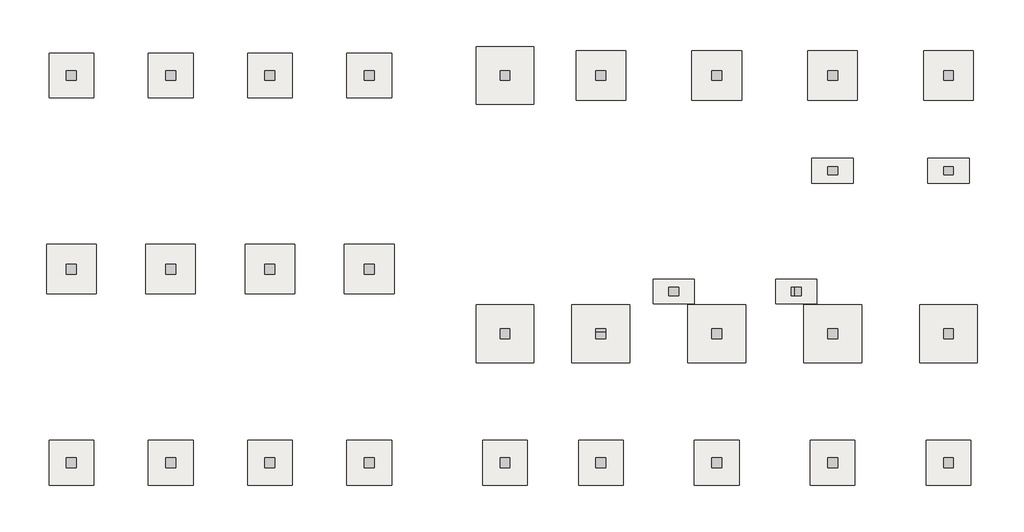
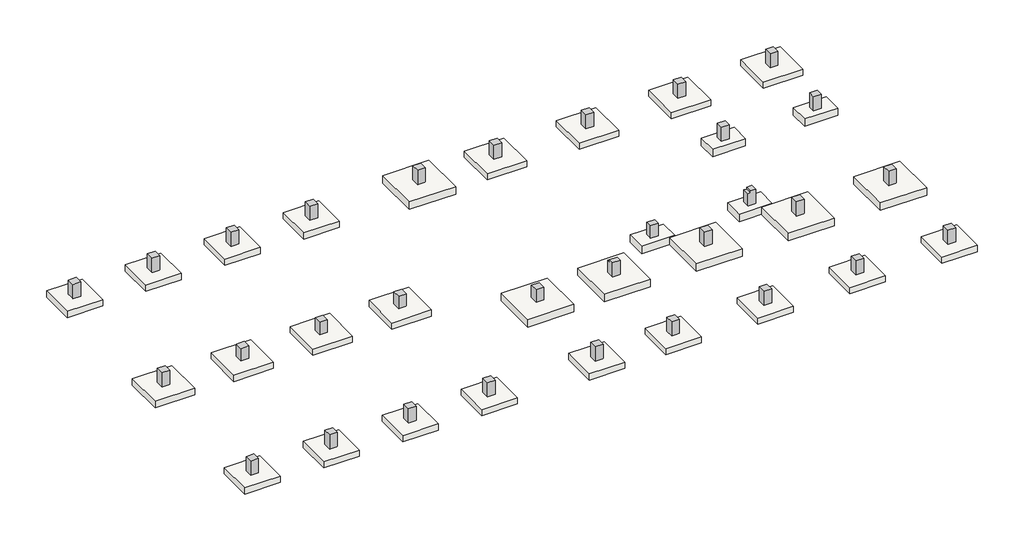
# Not in any storey: 31 columns, 31 slabs.
# Revit data of these elements (continued)
# Type "Foundation Rectangular (Non-Pile) : H_SF_AR_S18_W2700xL2700xT500_Bitumen_F1" (continued)
#   H_WM Code_1 = "A03AD032-00010 |  | M3 | Concrete Work | Substructure Work | Structural Concrete | Cement Type-1 | 20MPa < F'c (Cylinder Strength) ≤ 25MPa |  |  |  | A03AD032-00010 Concrete Work Substructure Work Structural Concrete  Cement Type-1 20MPa < F'c (Cylinder Strength) ≤ 25MPa      |  F'c (Cylinder Strength) = 24MPa"
#   H_WM Code_2 = "A03AD037-00002 |  | TON | Concrete Work | Substructure Work | Rebar Work | Deformed Bar (Non-Coat.) | 400MPa<Fy≤470MPa |  |  |  | A03AD037-00002 Concrete Work Substructure Work Rebar Work Deformed Bar (Non-Coat.)  400MPa<Fy≤470MPa      | ASTM A615 GRADE 60 (Fy=420MPa)"
#   H_WM Code_3 = "A03AD035-00001 |  | M2 | Concrete Work | Substructure Work | Form Work (3 times in use) | Flat Form | Dressed Lumber, Plywood or Steel Form(Wood Planks are not Allowed) incl. Chamfer |  |  | A03AD035-00001 Concrete Work Substructure Work Form Work (3 times in use) Flat Form     Dressed Lumber, Plywood or Steel Form(Wood Planks are not Allowed) incl. Chamfer   |"
#   H_WM Code_4 = "A03AH056-00001 |  | M2 | Concrete Work | Concrete Protective Coating (U/G) | Bitumen/Bituminous/Asphalt Coating |  | A03AH056-00001 Concrete Work Concrete Protective Coating (U/G) Bitumen/Bituminous/Asphalt Coating         |"
#   H_WM Code_5 = "A01ZZ001-00004 |  | M3 | Earth Work | - | Excavation | Soil, Mech. |  | D ≤ 2.0M |  |  | A01ZZ001-00004 Earth Work - Excavation Soil, Mech.      D ≤ 2.0M  | D=2.0m"
#   H_WM Code_6 = "A01ZZ003-00001 |  | M3 | Earth Work | - | Backfill | Re-use, Soil |  |  |  | Compaction=(  )% | A01ZZ003-00001 Earth Work - Backfill Re-use, Soil        | Compaction=( 95 )%"
#   H_WM Code_7 = "A01ZZ004-00001 |  | M3 | Earth Work | - | Disposal | Soil |  |  |  | Disposal Distance=Appx. (  )km from Site | A01ZZ004-00001 Earth Work - Disposal Soil        | Disposal Distance=Appx. (20 )km from Site"
#   Top bar = "D25@300"
#   Description = "UG Shallow Foundation"
#   Bottom bar = "D20@300"
#   Width = 2700 mm
#   Length = 2700 mm
#   Foundation Thickness = 500 mm
#   Structural Material [instance default] = none
#   Assembly Code = ""
# Type "Foundation Rectangular (Non-Pile) : H_SF_AR_S18_W3500xL3500xT600_Bitumen_F3"
#   H_Q'ty Cal Type Tag = "SF-Q4"
#   H_WM Code_1 = "A03AD032-00010 |  | M3 | Concrete Work | Substructure Work | Structural Concrete | Cement Type-1 | 20MPa < F'c (Cylinder Strength) ≤ 25MPa |  |  |  | A03AD032-00010 Concrete Work Substructure Work Structural Concrete  Cement Type-1 20MPa < F'c (Cylinder Strength) ≤ 25MPa      |  F'c (Cylinder Strength) = 24MPa"
#   H_WM Code_2 = "A03AD037-00002 |  | TON | Concrete Work | Substructure Work | Rebar Work | Deformed Bar (Non-Coat.) | 400MPa<Fy≤470MPa |  |  |  | A03AD037-00002 Concrete Work Substructure Work Rebar Work Deformed Bar (Non-Coat.)  400MPa<Fy≤470MPa      | ASTM A615 GRADE 60 (Fy=420MPa)"
#   H_WM Code_3 = "A03AD035-00001 |  | M2 | Concrete Work | Substructure Work | Form Work (3 times in use) | Flat Form | Dressed Lumber, Plywood or Steel Form(Wood Planks are not Allowed) incl. Chamfer |  |  | A03AD035-00001 Concrete Work Substructure Work Form Work (3 times in use) Flat Form     Dressed Lumber, Plywood or Steel Form(Wood Planks are not Allowed) incl. Chamfer   |"
#   H_WM Code_4 = "A03AH056-00001 |  | M2 | Concrete Work | Concrete Protective Coating (U/G) | Bitumen/Bituminous/Asphalt Coating |  | A03AH056-00001 Concrete Work Concrete Protective Coating (U/G) Bitumen/Bituminous/Asphalt Coating         |"
#   H_WM Code_5 = "A01ZZ001-00004 |  | M3 | Earth Work | - | Excavation | Soil, Mech. |  | D ≤ 2.0M |  |  | A01ZZ001-00004 Earth Work - Excavation Soil, Mech.      D ≤ 2.0M  | D=2.0m"
#   H_WM Code_6 = "A01ZZ003-00001 |  | M3 | Earth Work | - | Backfill | Re-use, Soil |  |  |  | Compaction=(  )% | A01ZZ003-00001 Earth Work - Backfill Re-use, Soil        | Compaction=( 95 )%"
#   H_WM Code_7 = "A01ZZ004-00001 |  | M3 | Earth Work | - | Disposal | Soil |  |  |  | Disposal Distance=Appx. (  )km from Site | A01ZZ004-00001 Earth Work - Disposal Soil        | Disposal Distance=Appx. (20 )km from Site"
#   Top bar = "D25@300"
#   Description = "UG Shallow Foundation"
#   Bottom bar = "D20@300"
#   Width = 3500 mm
#   Length = 3500 mm
#   Foundation Thickness = 600 mm
#   Structural Material [instance default] = none
#   Assembly Code = ""
# Type "Foundation Rectangular (Non-Pile) : H_SF_AR_S18_W3000xL3000xT500_Bitumen_F2A"
#   H_Q'ty Cal Type Tag = "SF-Q4"
#   H_WM Code_1 = "A03AD032-00010 |  | M3 | Concrete Work | Substructure Work | Structural Concrete | Cement Type-1 | 20MPa < F'c (Cylinder Strength) ≤ 25MPa |  |  |  | A03AD032-00010 Concrete Work Substructure Work Structural Concrete  Cement Type-1 20MPa < F'c (Cylinder Strength) ≤ 25MPa      |  F'c (Cylinder Strength) = 24MPa"
#   H_WM Code_2 = "A03AD037-00002 |  | TON | Concrete Work | Substructure Work | Rebar Work | Deformed Bar (Non-Coat.) | 400MPa<Fy≤470MPa |  |  |  | A03AD037-00002 Concrete Work Substructure Work Rebar Work Deformed Bar (Non-Coat.)  400MPa<Fy≤470MPa      | ASTM A615 GRADE 60 (Fy=420MPa)"
#   H_WM Code_3 = "A03AD035-00001 |  | M2 | Concrete Work | Substructure Work | Form Work (3 times in use) | Flat Form | Dressed Lumber, Plywood or Steel Form(Wood Planks are not Allowed) incl. Chamfer |  |  | A03AD035-00001 Concrete Work Substructure Work Form Work (3 times in use) Flat Form     Dressed Lumber, Plywood or Steel Form(Wood Planks are not Allowed) incl. Chamfer   |"
#   H_WM Code_4 = "A03AH056-00001 |  | M2 | Concrete Work | Concrete Protective Coating (U/G) | Bitumen/Bituminous/Asphalt Coating |  | A03AH056-00001 Concrete Work Concrete Protective Coating (U/G) Bitumen/Bituminous/Asphalt Coating         |"
#   H_WM Code_5 = "A01ZZ001-00004 |  | M3 | Earth Work | - | Excavation | Soil, Mech. |  | D ≤ 2.0M |  |  | A01ZZ001-00004 Earth Work - Excavation Soil, Mech.      D ≤ 2.0M  | D=2.0m"
#   H_WM Code_6 = "A01ZZ003-00001 |  | M3 | Earth Work | - | Backfill | Re-use, Soil |  |  |  | Compaction=(  )% | A01ZZ003-00001 Earth Work - Backfill Re-use, Soil        | Compaction=( 95 )%"
#   H_WM Code_7 = "A01ZZ004-00001 |  | M3 | Earth Work | - | Disposal | Soil |  |  |  | Disposal Distance=Appx. (  )km from Site | A01ZZ004-00001 Earth Work - Disposal Soil        | Disposal Distance=Appx. (20 )km from Site"
#   Top bar = "D25@300"
#   Description = "UG Shallow Foundation"
#   Bottom bar = "D20@300"
#   Width = 3000 mm
#   Length = 3000 mm
#   Foundation Thickness = 500 mm
#   Structural Material [instance default] = none
#   Assembly Code = ""
# Type "Foundation Rectangular (Non-Pile) : H_SF_AR_S18_W2700xL2700xT500_Bitumen_F1A"
#   H_Q'ty Cal Type Tag = "SF-Q4"
#   H_WM Code_1 = "A03AD032-00010 |  | M3 | Concrete Work | Substructure Work | Structural Concrete | Cement Type-1 | 20MPa < F'c (Cylinder Strength) ≤ 25MPa |  |  |  | A03AD032-00010 Concrete Work Substructure Work Structural Concrete  Cement Type-1 20MPa < F'c (Cylinder Strength) ≤ 25MPa      |  F'c (Cylinder Strength) = 24MPa"
#   H_WM Code_2 = "A03AD037-00002 |  | TON | Concrete Work | Substructure Work | Rebar Work | Deformed Bar (Non-Coat.) | 400MPa<Fy≤470MPa |  |  |  | A03AD037-00002 Concrete Work Substructure Work Rebar Work Deformed Bar (Non-Coat.)  400MPa<Fy≤470MPa      | ASTM A615 GRADE 60 (Fy=420MPa)"
#   H_WM Code_3 = "A03AD035-00001 |  | M2 | Concrete Work | Substructure Work | Form Work (3 times in use) | Flat Form | Dressed Lumber, Plywood or Steel Form(Wood Planks are not Allowed) incl. Chamfer |  |  | A03AD035-00001 Concrete Work Substructure Work Form Work (3 times in use) Flat Form     Dressed Lumber, Plywood or Steel Form(Wood Planks are not Allowed) incl. Chamfer   |"
#   H_WM Code_4 = "A03AH056-00001 |  | M2 | Concrete Work | Concrete Protective Coating (U/G) | Bitumen/Bituminous/Asphalt Coating |  | A03AH056-00001 Concrete Work Concrete Protective Coating (U/G) Bitumen/Bituminous/Asphalt Coating         |"
#   H_WM Code_5 = "A01ZZ001-00004 |  | M3 | Earth Work | - | Excavation | Soil, Mech. |  | D ≤ 2.0M |  |  | A01ZZ001-00004 Earth Work - Excavation Soil, Mech.      D ≤ 2.0M  | D=2.0m"
#   H_WM Code_6 = "A01ZZ003-00001 |  | M3 | Earth Work | - | Backfill | Re-use, Soil |  |  |  | Compaction=(  )% | A01ZZ003-00001 Earth Work - Backfill Re-use, Soil        | Compaction=( 95 )%"
#   H_WM Code_7 = "A01ZZ004-00001 |  | M3 | Earth Work | - | Disposal | Soil |  |  |  | Disposal Distance=Appx. (  )km from Site | A01ZZ004-00001 Earth Work - Disposal Soil        | Disposal Distance=Appx. (20 )km from Site"
#   Top bar = "D25@300"
#   Description = "UG Shallow Foundation"
#   Bottom bar = "D20@300"
#   Width = 2700 mm
#   Length = 2700 mm
#   Foundation Thickness = 500 mm
#   Structural Material [instance default] = none
#   Assembly Code = ""
# Type "Foundation Rectangular (Non-Pile) : H_SF_AR_S18_W2500xL1500xT600_Bitumen_F4"
#   H_Q'ty Cal Type Tag = "SF-Q4"
#   H_WM Code_1 = "A03AD032-00010 |  | M3 | Concrete Work | Substructure Work | Structural Concrete | Cement Type-1 | 20MPa < F'c (Cylinder Strength) ≤ 25MPa |  |  |  | A03AD032-00010 Concrete Work Substructure Work Structural Concrete  Cement Type-1 20MPa < F'c (Cylinder Strength) ≤ 25MPa      |  F'c (Cylinder Strength) = 24MPa"
#   H_WM Code_2 = "A03AD037-00002 |  | TON | Concrete Work | Substructure Work | Rebar Work | Deformed Bar (Non-Coat.) | 400MPa<Fy≤470MPa |  |  |  | A03AD037-00002 Concrete Work Substructure Work Rebar Work Deformed Bar (Non-Coat.)  400MPa<Fy≤470MPa      | ASTM A615 GRADE 60 (Fy=420MPa)"
#   H_WM Code_3 = "A03AD035-00001 |  | M2 | Concrete Work | Substructure Work | Form Work (3 times in use) | Flat Form | Dressed Lumber, Plywood or Steel Form(Wood Planks are not Allowed) incl. Chamfer |  |  | A03AD035-00001 Concrete Work Substructure Work Form Work (3 times in use) Flat Form     Dressed Lumber, Plywood or Steel Form(Wood Planks are not Allowed) incl. Chamfer   |"
#   H_WM Code_4 = "A03AH056-00001 |  | M2 | Concrete Work | Concrete Protective Coating (U/G) | Bitumen/Bituminous/Asphalt Coating |  | A03AH056-00001 Concrete Work Concrete Protective Coating (U/G) Bitumen/Bituminous/Asphalt Coating         |"
#   H_WM Code_5 = "A01ZZ001-00004 |  | M3 | Earth Work | - | Excavation | Soil, Mech. |  | D ≤ 2.0M |  |  | A01ZZ001-00004 Earth Work - Excavation Soil, Mech.      D ≤ 2.0M  | D=2.0m"
#   H_WM Code_6 = "A01ZZ003-00001 |  | M3 | Earth Work | - | Backfill | Re-use, Soil |  |  |  | Compaction=(  )% | A01ZZ003-00001 Earth Work - Backfill Re-use, Soil        | Compaction=( 95 )%"
#   H_WM Code_7 = "A01ZZ004-00001 |  | M3 | Earth Work | - | Disposal | Soil |  |  |  | Disposal Distance=Appx. (  )km from Site | A01ZZ004-00001 Earth Work - Disposal Soil        | Disposal Distance=Appx. (20 )km from Site"
#   Top bar = "D25@300"
#   Description = "UG Shallow Foundation"
#   Bottom bar = "D20@300"
#   Width = 2500 mm
#   Length = 1500 mm
#   Foundation Thickness = 600 mm
#   Structural Material [instance default] = none
#   Assembly Code = ""
# Elements 1, 2, 3, 4, 5, 6, 7, 8, 9, 10, 11, 12, 13, 14, 15, 16, 17, 18, 19, 20, 21, 22, 23, 24, 25, 26, 27 (IfcColumn, "RC_Column_Rectangular : H_SC_AR_S15_UG PED_W600xL600_Bit")
#   Comments = ""
#   hec_material3 = none
#   hec_material2 = none
#   hec_material1 = none
#   Structural Material = Concrete - Cast-in-Place Concrete - 35 MPa
#   Phase Created = New Construction
#   Materials on its faces: "Concrete - Cast-in-Place Concrete - 35 MPa"
# Elements 28, 29, 30, 31 (IfcColumn, "RC_Column_Rectangular : H_SC_AR_S15_UG PED_W600xL500_Bit_PD1A")
#   Comments = ""
#   hec_material3 = none
#   hec_material2 = none
#   hec_material1 = none
#   Structural Material = Concrete - Cast-in-Place Concrete - 35 MPa
#   Phase Created = New Construction
#   Materials on its faces: "Concrete - Cast-in-Place Concrete - 35 MPa"
# Elements 32, 33, 34, 35 (IfcSlab, "Foundation Rectangular (Non-Pile) : H_SF_AR_S18_W3000xL3000xT500_Bitumen_F2")
#   Comments = ""
#   Structural Material = none
#   Phase Created = New Construction
# Elements 36, 37, 38, 39, 51, 52, 53, 56, 57, 58 (IfcSlab, "Foundation Rectangular (Non-Pile) : H_SF_AR_S18_W2700xL2700xT500_Bitumen_F1")
#   Comments = ""
#   Structural Material = none
#   Phase Created = New Construction
# Elements 40, 45, 46, 47, 48, 49 (IfcSlab, "Foundation Rectangular (Non-Pile) : H_SF_AR_S18_W3500xL3500xT600_Bitumen_F3")
#   Comments = ""
#   Structural Material = none
#   Phase Created = New Construction
# Elements 41, 42, 43, 44 (IfcSlab, "Foundation Rectangular (Non-Pile) : H_SF_AR_S18_W3000xL3000xT500_Bitumen_F2A")
#   Comments = ""
#   Structural Material = none
#   Phase Created = New Construction
# Elements 50, 54, 55 (IfcSlab, "Foundation Rectangular (Non-Pile) : H_SF_AR_S18_W2700xL2700xT500_Bitumen_F1A")
#   Comments = ""
#   Structural Material = none
#   Phase Created = New Construction
# Elements 59, 60, 61, 62 (IfcSlab, "Foundation Rectangular (Non-Pile) : H_SF_AR_S18_W2500xL1500xT600_Bitumen_F4")
#   Comments = ""
#   Structural Material = none
#   Phase Created = New Construction
# Materials
#   "Concrete - Cast-in-Place Concrete - 35 MPa": class "Concrete", colour RGB 192 192 192, transparency 0, Description = "ACRYLIC EMULSION PAINT ON THK.13 CEMENT PLASTER", Cost = 0
